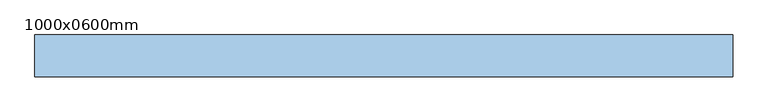
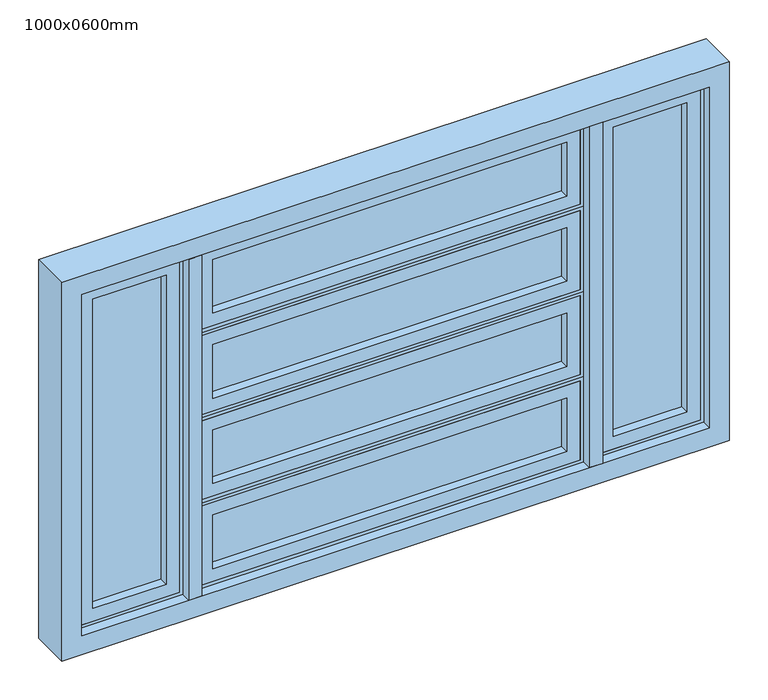
"""IFC4 building model written with IfcOpenShell, lengths in millimetres: window geometry, Janela Basculante 02 : 1000x0600mm."""

from ifc_helpers import new_model, si_unit, frame, origin, place, context, project, spatial, polyline, outline, extrude, faceted_brep, source, transform, mapped, element, save


def window_1000x0600mm_c1d4fbe1(model_context):
    return source(origin(), model_context, "Body", "SolidModel", [
        extrude(outline(polyline([(452.0, -29.6), (452.0, -36.6), (328.0, -36.6), (328.0, -29.6), (452.0, -29.6)])), frame((0.0, 0.0, 598.0), z_axis=(0.0, 0.0, 1.0), x_axis=(1.0, 0.0, 0.0)), (0.0, 0.0, 1.0), 504.0),
        faceted_brep([(335.0, -50.6, 1095.0), (335.0, -50.6, 605.0), (335.0, -36.6, 605.0), (335.0, -36.6, 1095.0), (328.0, -36.6, 1102.0), (328.0, -36.6, 598.0), (328.0, -29.6, 598.0), (328.0, -29.6, 1102.0), (335.0, -29.6, 1095.0), (335.0, -29.6, 605.0), (335.0, -15.6, 605.0), (335.0, -15.6, 1095.0), (315.0, -15.6, 1115.0), (315.0, -15.6, 585.0), (315.0, -50.6, 585.0), (315.0, -50.6, 1115.0), (445.0, -50.6, 605.0), (445.0, -36.6, 605.0), (452.0, -36.6, 598.0), (452.0, -29.6, 598.0), (445.0, -29.6, 605.0), (445.0, -15.6, 605.0), (465.0, -15.6, 585.0), (465.0, -50.6, 585.0), (445.0, -50.6, 1095.0), (445.0, -36.6, 1095.0), (452.0, -36.6, 1102.0), (452.0, -29.6, 1102.0), (445.0, -29.6, 1095.0), (445.0, -15.6, 1095.0), (465.0, -15.6, 1115.0), (465.0, -50.6, 1115.0)], [[[0, 1, 2, 3]], [[4, 5, 6, 7]], [[8, 9, 10, 11]], [[12, 13, 14, 15]], [[1, 16, 17, 2]], [[5, 18, 19, 6]], [[9, 20, 21, 10]], [[13, 22, 23, 14]], [[16, 24, 25, 17]], [[18, 26, 27, 19]], [[20, 28, 29, 21]], [[22, 30, 31, 23]], [[15, 14, 23, 31], [1, 0, 24, 16]], [[24, 0, 3, 25]], [[5, 4, 26, 18], [3, 2, 17, 25]], [[26, 4, 7, 27]], [[7, 6, 19, 27], [9, 8, 28, 20]], [[28, 8, 11, 29]], [[13, 12, 30, 22], [11, 10, 21, 29]], [[30, 12, 15, 31]]]),
        faceted_brep([(315.0, -50.6, 1115.0), (315.0, -50.6, 585.0), (315.0, -15.6, 585.0), (315.0, -15.6, 1115.0), (320.0, -15.6, 1110.0), (320.0, -15.6, 590.0), (320.0, -10.6, 590.0), (320.0, -10.6, 1110.0), (310.0, -10.6, 1120.0), (310.0, -10.6, 580.0), (310.0, -50.6, 580.0), (310.0, -50.6, 1120.0), (465.0, -50.6, 585.0), (465.0, -15.6, 585.0), (460.0, -15.6, 590.0), (460.0, -10.6, 590.0), (470.0, -10.6, 580.0), (470.0, -50.6, 580.0), (465.0, -50.6, 1115.0), (465.0, -15.6, 1115.0), (460.0, -15.6, 1110.0), (460.0, -10.6, 1110.0), (470.0, -10.6, 1120.0), (470.0, -50.6, 1120.0)], [[[0, 1, 2, 3]], [[4, 5, 6, 7]], [[8, 9, 10, 11]], [[1, 12, 13, 2]], [[5, 14, 15, 6]], [[9, 16, 17, 10]], [[12, 18, 19, 13]], [[14, 20, 21, 15]], [[16, 22, 23, 17]], [[11, 10, 17, 23], [1, 0, 18, 12]], [[18, 0, 3, 19]], [[3, 2, 13, 19], [5, 4, 20, 14]], [[20, 4, 7, 21]], [[9, 8, 22, 16], [7, 6, 15, 21]], [[22, 8, 11, 23]]]),
        extrude(outline(polyline([(-452.0, -29.6), (-328.0, -29.6), (-328.0, -36.6), (-452.0, -36.6), (-452.0, -29.6)])), frame((0.0, 0.0, 598.0), z_axis=(0.0, 0.0, 1.0), x_axis=(1.0, 0.0, 0.0)), (0.0, 0.0, 1.0), 504.0),
        faceted_brep([(-335.0, -50.6, 1095.0), (-335.0, -36.6, 1095.0), (-335.0, -36.6, 605.0), (-335.0, -50.6, 605.0), (-328.0, -36.6, 1102.0), (-328.0, -29.6, 1102.0), (-328.0, -29.6, 598.0), (-328.0, -36.6, 598.0), (-335.0, -29.6, 1095.0), (-335.0, -15.6, 1095.0), (-335.0, -15.6, 605.0), (-335.0, -29.6, 605.0), (-315.0, -15.6, 1115.0), (-315.0, -50.6, 1115.0), (-315.0, -50.6, 585.0), (-315.0, -15.6, 585.0), (-445.0, -36.6, 605.0), (-445.0, -50.6, 605.0), (-452.0, -29.6, 598.0), (-452.0, -36.6, 598.0), (-445.0, -15.6, 605.0), (-445.0, -29.6, 605.0), (-465.0, -50.6, 585.0), (-465.0, -15.6, 585.0), (-445.0, -36.6, 1095.0), (-445.0, -50.6, 1095.0), (-452.0, -29.6, 1102.0), (-452.0, -36.6, 1102.0), (-445.0, -15.6, 1095.0), (-445.0, -29.6, 1095.0), (-465.0, -50.6, 1115.0), (-465.0, -15.6, 1115.0)], [[[0, 1, 2, 3]], [[4, 5, 6, 7]], [[8, 9, 10, 11]], [[12, 13, 14, 15]], [[3, 2, 16, 17]], [[7, 6, 18, 19]], [[11, 10, 20, 21]], [[15, 14, 22, 23]], [[17, 16, 24, 25]], [[19, 18, 26, 27]], [[21, 20, 28, 29]], [[23, 22, 30, 31]], [[13, 30, 22, 14], [3, 17, 25, 0]], [[25, 24, 1, 0]], [[7, 19, 27, 4], [1, 24, 16, 2]], [[27, 26, 5, 4]], [[5, 26, 18, 6], [11, 21, 29, 8]], [[29, 28, 9, 8]], [[15, 23, 31, 12], [9, 28, 20, 10]], [[31, 30, 13, 12]]]),
        faceted_brep([(-315.0, -50.6, 1115.0), (-315.0, -15.6, 1115.0), (-315.0, -15.6, 585.0), (-315.0, -50.6, 585.0), (-320.0, -15.6, 1110.0), (-320.0, -10.6, 1110.0), (-320.0, -10.6, 590.0), (-320.0, -15.6, 590.0), (-310.0, -10.6, 1120.0), (-310.0, -50.6, 1120.0), (-310.0, -50.6, 580.0), (-310.0, -10.6, 580.0), (-465.0, -15.6, 585.0), (-465.0, -50.6, 585.0), (-460.0, -10.6, 590.0), (-460.0, -15.6, 590.0), (-470.0, -50.6, 580.0), (-470.0, -10.6, 580.0), (-465.0, -15.6, 1115.0), (-465.0, -50.6, 1115.0), (-460.0, -10.6, 1110.0), (-460.0, -15.6, 1110.0), (-470.0, -50.6, 1120.0), (-470.0, -10.6, 1120.0)], [[[0, 1, 2, 3]], [[4, 5, 6, 7]], [[8, 9, 10, 11]], [[3, 2, 12, 13]], [[7, 6, 14, 15]], [[11, 10, 16, 17]], [[13, 12, 18, 19]], [[15, 14, 20, 21]], [[17, 16, 22, 23]], [[9, 22, 16, 10], [3, 13, 19, 0]], [[19, 18, 1, 0]], [[1, 18, 12, 2], [7, 15, 21, 4]], [[21, 20, 5, 4]], [[11, 17, 23, 8], [5, 20, 14, 6]], [[23, 22, 9, 8]]]),
        extrude(outline(polyline([(-272.0, -29.6), (272.0, -29.6), (272.0, -36.6), (-272.0, -36.6), (-272.0, -29.6)])), frame((0.0, 0.0, 1003.0), z_axis=(0.0, 0.0, 1.0), x_axis=(1.0, 0.0, 0.0)), (0.0, 0.0, 1.0), 99.0),
        faceted_brep([(265.0, -50.6, 1095.0), (265.0, -36.6, 1095.0), (265.0, -36.6, 1010.0), (265.0, -50.6, 1010.0), (272.0, -36.6, 1102.0), (272.0, -29.6, 1102.0), (272.0, -29.6, 1003.0), (272.0, -36.6, 1003.0), (265.0, -29.6, 1095.0), (265.0, -15.6, 1095.0), (265.0, -15.6, 1010.0), (265.0, -29.6, 1010.0), (285.0, -15.6, 1115.0), (285.0, -50.6, 1115.0), (285.0, -50.6, 990.0), (285.0, -15.6, 990.0), (-265.0, -36.6, 1010.0), (-265.0, -50.6, 1010.0), (-272.0, -29.6, 1003.0), (-272.0, -36.6, 1003.0), (-265.0, -15.6, 1010.0), (-265.0, -29.6, 1010.0), (-285.0, -50.6, 990.0), (-285.0, -15.6, 990.0), (-265.0, -36.6, 1095.0), (-265.0, -50.6, 1095.0), (-272.0, -29.6, 1102.0), (-272.0, -36.6, 1102.0), (-265.0, -15.6, 1095.0), (-265.0, -29.6, 1095.0), (-285.0, -50.6, 1115.0), (-285.0, -15.6, 1115.0)], [[[0, 1, 2, 3]], [[4, 5, 6, 7]], [[8, 9, 10, 11]], [[12, 13, 14, 15]], [[3, 2, 16, 17]], [[7, 6, 18, 19]], [[11, 10, 20, 21]], [[15, 14, 22, 23]], [[17, 16, 24, 25]], [[19, 18, 26, 27]], [[21, 20, 28, 29]], [[23, 22, 30, 31]], [[13, 30, 22, 14], [3, 17, 25, 0]], [[25, 24, 1, 0]], [[7, 19, 27, 4], [1, 24, 16, 2]], [[27, 26, 5, 4]], [[5, 26, 18, 6], [11, 21, 29, 8]], [[29, 28, 9, 8]], [[15, 23, 31, 12], [9, 28, 20, 10]], [[31, 30, 13, 12]]]),
        faceted_brep([(285.0, -50.6, 1115.0), (285.0, -15.6, 1115.0), (285.0, -15.6, 990.0), (285.0, -50.6, 990.0), (280.0, -15.6, 1110.0), (280.0, -10.6, 1110.0), (280.0, -10.6, 995.0), (280.0, -15.6, 995.0), (290.0, -10.6, 1120.0), (290.0, -50.6, 1120.0), (290.0, -50.6, 985.0), (290.0, -10.6, 985.0), (-285.0, -15.6, 990.0), (-285.0, -50.6, 990.0), (-280.0, -10.6, 995.0), (-280.0, -15.6, 995.0), (-290.0, -50.6, 985.0), (-290.0, -10.6, 985.0), (-285.0, -15.6, 1115.0), (-285.0, -50.6, 1115.0), (-280.0, -10.6, 1110.0), (-280.0, -15.6, 1110.0), (-290.0, -50.6, 1120.0), (-290.0, -10.6, 1120.0)], [[[0, 1, 2, 3]], [[4, 5, 6, 7]], [[8, 9, 10, 11]], [[3, 2, 12, 13]], [[7, 6, 14, 15]], [[11, 10, 16, 17]], [[13, 12, 18, 19]], [[15, 14, 20, 21]], [[17, 16, 22, 23]], [[9, 22, 16, 10], [3, 13, 19, 0]], [[19, 18, 1, 0]], [[1, 18, 12, 2], [7, 15, 21, 4]], [[21, 20, 5, 4]], [[11, 17, 23, 8], [5, 20, 14, 6]], [[23, 22, 9, 8]]]),
        extrude(outline(polyline([(-272.0, -29.6), (272.0, -29.6), (272.0, -36.6), (-272.0, -36.6), (-272.0, -29.6)])), frame((0.0, 0.0, 868.0), z_axis=(0.0, 0.0, 1.0), x_axis=(1.0, 0.0, 0.0)), (0.0, 0.0, 1.0), 99.0),
        faceted_brep([(265.0, -50.6, 960.0), (265.0, -36.6, 960.0), (265.0, -36.6, 875.0), (265.0, -50.6, 875.0), (272.0, -36.6, 967.0), (272.0, -29.6, 967.0), (272.0, -29.6, 868.0), (272.0, -36.6, 868.0), (265.0, -29.6, 960.0), (265.0, -15.6, 960.0), (265.0, -15.6, 875.0), (265.0, -29.6, 875.0), (285.0, -15.6, 980.0), (285.0, -50.6, 980.0), (285.0, -50.6, 855.0), (285.0, -15.6, 855.0), (-265.0, -36.6, 875.0), (-265.0, -50.6, 875.0), (-272.0, -29.6, 868.0), (-272.0, -36.6, 868.0), (-265.0, -15.6, 875.0), (-265.0, -29.6, 875.0), (-285.0, -50.6, 855.0), (-285.0, -15.6, 855.0), (-265.0, -36.6, 960.0), (-265.0, -50.6, 960.0), (-272.0, -29.6, 967.0), (-272.0, -36.6, 967.0), (-265.0, -15.6, 960.0), (-265.0, -29.6, 960.0), (-285.0, -50.6, 980.0), (-285.0, -15.6, 980.0)], [[[0, 1, 2, 3]], [[4, 5, 6, 7]], [[8, 9, 10, 11]], [[12, 13, 14, 15]], [[3, 2, 16, 17]], [[7, 6, 18, 19]], [[11, 10, 20, 21]], [[15, 14, 22, 23]], [[17, 16, 24, 25]], [[19, 18, 26, 27]], [[21, 20, 28, 29]], [[23, 22, 30, 31]], [[13, 30, 22, 14], [3, 17, 25, 0]], [[25, 24, 1, 0]], [[7, 19, 27, 4], [1, 24, 16, 2]], [[27, 26, 5, 4]], [[5, 26, 18, 6], [11, 21, 29, 8]], [[29, 28, 9, 8]], [[15, 23, 31, 12], [9, 28, 20, 10]], [[31, 30, 13, 12]]]),
        faceted_brep([(285.0, -50.6, 980.0), (285.0, -15.6, 980.0), (285.0, -15.6, 855.0), (285.0, -50.6, 855.0), (280.0, -15.6, 975.0), (280.0, -10.6, 975.0), (280.0, -10.6, 860.0), (280.0, -15.6, 860.0), (290.0, -10.6, 985.0), (290.0, -50.6, 985.0), (290.0, -50.6, 850.0), (290.0, -10.6, 850.0), (-285.0, -15.6, 855.0), (-285.0, -50.6, 855.0), (-280.0, -10.6, 860.0), (-280.0, -15.6, 860.0), (-290.0, -50.6, 850.0), (-290.0, -10.6, 850.0), (-285.0, -15.6, 980.0), (-285.0, -50.6, 980.0), (-280.0, -10.6, 975.0), (-280.0, -15.6, 975.0), (-290.0, -50.6, 985.0), (-290.0, -10.6, 985.0)], [[[0, 1, 2, 3]], [[4, 5, 6, 7]], [[8, 9, 10, 11]], [[3, 2, 12, 13]], [[7, 6, 14, 15]], [[11, 10, 16, 17]], [[13, 12, 18, 19]], [[15, 14, 20, 21]], [[17, 16, 22, 23]], [[9, 22, 16, 10], [3, 13, 19, 0]], [[19, 18, 1, 0]], [[1, 18, 12, 2], [7, 15, 21, 4]], [[21, 20, 5, 4]], [[11, 17, 23, 8], [5, 20, 14, 6]], [[23, 22, 9, 8]]]),
        extrude(outline(polyline([(-272.0, -29.6), (272.0, -29.6), (272.0, -36.6), (-272.0, -36.6), (-272.0, -29.6)])), frame((0.0, 0.0, 733.0), z_axis=(0.0, 0.0, 1.0), x_axis=(1.0, 0.0, 0.0)), (0.0, 0.0, 1.0), 99.0),
        faceted_brep([(265.0, -50.6, 825.0), (265.0, -36.6, 825.0), (265.0, -36.6, 740.0), (265.0, -50.6, 740.0), (272.0, -36.6, 832.0), (272.0, -29.6, 832.0), (272.0, -29.6, 733.0), (272.0, -36.6, 733.0), (265.0, -29.6, 825.0), (265.0, -15.6, 825.0), (265.0, -15.6, 740.0), (265.0, -29.6, 740.0), (285.0, -15.6, 845.0), (285.0, -50.6, 845.0), (285.0, -50.6, 720.0), (285.0, -15.6, 720.0), (-265.0, -36.6, 740.0), (-265.0, -50.6, 740.0), (-272.0, -29.6, 733.0), (-272.0, -36.6, 733.0), (-265.0, -15.6, 740.0), (-265.0, -29.6, 740.0), (-285.0, -50.6, 720.0), (-285.0, -15.6, 720.0), (-265.0, -36.6, 825.0), (-265.0, -50.6, 825.0), (-272.0, -29.6, 832.0), (-272.0, -36.6, 832.0), (-265.0, -15.6, 825.0), (-265.0, -29.6, 825.0), (-285.0, -50.6, 845.0), (-285.0, -15.6, 845.0)], [[[0, 1, 2, 3]], [[4, 5, 6, 7]], [[8, 9, 10, 11]], [[12, 13, 14, 15]], [[3, 2, 16, 17]], [[7, 6, 18, 19]], [[11, 10, 20, 21]], [[15, 14, 22, 23]], [[17, 16, 24, 25]], [[19, 18, 26, 27]], [[21, 20, 28, 29]], [[23, 22, 30, 31]], [[13, 30, 22, 14], [3, 17, 25, 0]], [[25, 24, 1, 0]], [[7, 19, 27, 4], [1, 24, 16, 2]], [[27, 26, 5, 4]], [[5, 26, 18, 6], [11, 21, 29, 8]], [[29, 28, 9, 8]], [[15, 23, 31, 12], [9, 28, 20, 10]], [[31, 30, 13, 12]]]),
        faceted_brep([(285.0, -50.6, 845.0), (285.0, -15.6, 845.0), (285.0, -15.6, 720.0), (285.0, -50.6, 720.0), (280.0, -15.6, 840.0), (280.0, -10.6, 840.0), (280.0, -10.6, 725.0), (280.0, -15.6, 725.0), (290.0, -10.6, 850.0), (290.0, -50.6, 850.0), (290.0, -50.6, 715.0), (290.0, -10.6, 715.0), (-285.0, -15.6, 720.0), (-285.0, -50.6, 720.0), (-280.0, -10.6, 725.0), (-280.0, -15.6, 725.0), (-290.0, -50.6, 715.0), (-290.0, -10.6, 715.0), (-285.0, -15.6, 845.0), (-285.0, -50.6, 845.0), (-280.0, -10.6, 840.0), (-280.0, -15.6, 840.0), (-290.0, -50.6, 850.0), (-290.0, -10.6, 850.0)], [[[0, 1, 2, 3]], [[4, 5, 6, 7]], [[8, 9, 10, 11]], [[3, 2, 12, 13]], [[7, 6, 14, 15]], [[11, 10, 16, 17]], [[13, 12, 18, 19]], [[15, 14, 20, 21]], [[17, 16, 22, 23]], [[9, 22, 16, 10], [3, 13, 19, 0]], [[19, 18, 1, 0]], [[1, 18, 12, 2], [7, 15, 21, 4]], [[21, 20, 5, 4]], [[11, 17, 23, 8], [5, 20, 14, 6]], [[23, 22, 9, 8]]]),
        extrude(outline(polyline([(-272.0, -29.6), (272.0, -29.6), (272.0, -36.6), (-272.0, -36.6), (-272.0, -29.6)])), frame((0.0, 0.0, 598.0), z_axis=(0.0, 0.0, 1.0), x_axis=(1.0, 0.0, 0.0)), (0.0, 0.0, 1.0), 99.0),
        faceted_brep([(265.0, -50.6, 690.0), (265.0, -36.6, 690.0), (265.0, -36.6, 605.0), (265.0, -50.6, 605.0), (272.0, -36.6, 697.0), (272.0, -29.6, 697.0), (272.0, -29.6, 598.0), (272.0, -36.6, 598.0), (265.0, -29.6, 690.0), (265.0, -15.6, 690.0), (265.0, -15.6, 605.0), (265.0, -29.6, 605.0), (285.0, -15.6, 710.0), (285.0, -50.6, 710.0), (285.0, -50.6, 585.0), (285.0, -15.6, 585.0), (-265.0, -36.6, 605.0), (-265.0, -50.6, 605.0), (-272.0, -29.6, 598.0), (-272.0, -36.6, 598.0), (-265.0, -15.6, 605.0), (-265.0, -29.6, 605.0), (-285.0, -50.6, 585.0), (-285.0, -15.6, 585.0), (-265.0, -36.6, 690.0), (-265.0, -50.6, 690.0), (-272.0, -29.6, 697.0), (-272.0, -36.6, 697.0), (-265.0, -15.6, 690.0), (-265.0, -29.6, 690.0), (-285.0, -50.6, 710.0), (-285.0, -15.6, 710.0)], [[[0, 1, 2, 3]], [[4, 5, 6, 7]], [[8, 9, 10, 11]], [[12, 13, 14, 15]], [[3, 2, 16, 17]], [[7, 6, 18, 19]], [[11, 10, 20, 21]], [[15, 14, 22, 23]], [[17, 16, 24, 25]], [[19, 18, 26, 27]], [[21, 20, 28, 29]], [[23, 22, 30, 31]], [[13, 30, 22, 14], [3, 17, 25, 0]], [[25, 24, 1, 0]], [[7, 19, 27, 4], [1, 24, 16, 2]], [[27, 26, 5, 4]], [[5, 26, 18, 6], [11, 21, 29, 8]], [[29, 28, 9, 8]], [[15, 23, 31, 12], [9, 28, 20, 10]], [[31, 30, 13, 12]]]),
        faceted_brep([(285.0, -50.6, 710.0), (285.0, -15.6, 710.0), (285.0, -15.6, 585.0), (285.0, -50.6, 585.0), (280.0, -15.6, 705.0), (280.0, -10.6, 705.0), (280.0, -10.6, 590.0), (280.0, -15.6, 590.0), (290.0, -10.6, 715.0), (290.0, -50.6, 715.0), (290.0, -50.6, 580.0), (290.0, -10.6, 580.0), (-285.0, -15.6, 585.0), (-285.0, -50.6, 585.0), (-280.0, -10.6, 590.0), (-280.0, -15.6, 590.0), (-290.0, -50.6, 580.0), (-290.0, -10.6, 580.0), (-285.0, -15.6, 710.0), (-285.0, -50.6, 710.0), (-280.0, -10.6, 705.0), (-280.0, -15.6, 705.0), (-290.0, -50.6, 715.0), (-290.0, -10.6, 715.0)], [[[0, 1, 2, 3]], [[4, 5, 6, 7]], [[8, 9, 10, 11]], [[3, 2, 12, 13]], [[7, 6, 14, 15]], [[11, 10, 16, 17]], [[13, 12, 18, 19]], [[15, 14, 20, 21]], [[17, 16, 22, 23]], [[9, 22, 16, 10], [3, 13, 19, 0]], [[19, 18, 1, 0]], [[1, 18, 12, 2], [7, 15, 21, 4]], [[21, 20, 5, 4]], [[11, 17, 23, 8], [5, 20, 14, 6]], [[23, 22, 9, 8]]]),
        extrude(outline(polyline([(290.0, -10.6), (310.0, -10.6), (310.0, -65.6), (290.0, -65.6), (290.0, -10.6)])), frame((0.0, 0.0, 580.0), z_axis=(0.0, 0.0, 1.0), x_axis=(1.0, 0.0, 0.0)), (0.0, 0.0, 1.0), 540.0),
        extrude(outline(polyline([(-310.0, -10.6), (-290.0, -10.6), (-290.0, -65.6), (-310.0, -65.6), (-310.0, -10.6)])), frame((0.0, 0.0, 580.0), z_axis=(0.0, 0.0, 1.0), x_axis=(1.0, 0.0, 0.0)), (0.0, 0.0, 1.0), 540.0),
        faceted_brep([(500.0, -5.6, 1150.0), (500.0, -65.6, 1150.0), (500.0, -65.6, 550.0), (500.0, -5.6, 550.0), (-500.0, -65.6, 1150.0), (-500.0, -65.6, 550.0), (470.0, -65.6, 580.0), (-470.0, -65.6, 580.0), (-470.0, -65.6, 1120.0), (470.0, -65.6, 1120.0), (-500.0, -5.6, 550.0), (-500.0, -5.6, 1150.0), (460.0, -5.6, 1110.0), (-460.0, -5.6, 1110.0), (-460.0, -5.6, 590.0), (460.0, -5.6, 590.0), (470.0, -10.6, 1120.0), (470.0, -10.6, 580.0), (-470.0, -10.6, 1120.0), (-470.0, -10.6, 580.0), (460.0, -10.6, 590.0), (-460.0, -10.6, 590.0), (-460.0, -10.6, 1110.0), (460.0, -10.6, 1110.0)], [[[0, 1, 2, 3]], [[1, 4, 5, 2], [6, 7, 8, 9]], [[3, 2, 5, 10]], [[3, 10, 11, 0], [12, 13, 14, 15]], [[9, 16, 17, 6]], [[16, 18, 19, 17], [20, 21, 22, 23]], [[6, 17, 19, 7]], [[10, 5, 4, 11]], [[7, 19, 18, 8]], [[23, 12, 15, 20]], [[20, 15, 14, 21]], [[21, 14, 13, 22]], [[11, 4, 1, 0]], [[8, 18, 16, 9]], [[22, 13, 12, 23]]]),
    ])


if __name__ == "__main__":
    model = new_model("IFC4")
    model_context = context("Model", 3, world=origin())
    ifc_project = project(units=[si_unit("LENGTHUNIT", "METRE", prefix="MILLI")], contexts=[model_context])
    site = spatial("IfcSite", under=ifc_project)
    building = spatial("IfcBuilding", under=site)
    placement = place(None, origin())
    window_1000x0600mm_shape = window_1000x0600mm_c1d4fbe1(model_context)
    element("IfcWindow", 1, ObjectType="Janela Basculante 02 : 1000x0600mm", at=placement, inside=building, context=model_context, shape_type="MappedRepresentation", body=[
        mapped(window_1000x0600mm_shape, transform((0.0, 0.0, 0.0), x_axis=(1.0, 0.0, 0.0), y_axis=(0.0, 1.0, 0.0), z_axis=(0.0, 0.0, 1.0))),
    ])
    save(model, "model.ifc")

# Revit data of these elements
# Type "Janela Basculante 02 : 1000x0600mm"
#   Type Mark = ""
#   SINAPI = ""
#   ref. v bascula = 13.50 cm
#   ref. h bascula = 58.00 cm
#   Ref. h basc lateral = 16.00 cm
#   Módulo Básico M = 10.00 cm
#   Largura de Coordenação Modular CM = 100.00 cm
#   Largura bascula lateral = 20.00 cm
#   Largura Batente = 6.00 cm
#   Altura de Coordenação Modular CM = 60.00 cm
#   Height = 60.00 cm
#   Altura Peitoril = 55.00 cm
#   Width = 100.00 cm
#   Altura Bascula Lateral = 54.00 cm
#   n° de basculas = 4
#   Número de Módulos Básicos nM Largura = 10
#   Número de Módulos Básicos nM Altura = 6
#   Material Quadro = Metal - Alumínio
#   Material Painel = Vidro
#   Wall Closure = (empty or 0)
#   Assembly Code = ""
# Element 1 (IfcWindow, "Janela Basculante 02 : 1000x0600mm")
#   Materials on its faces: "Metal - Alumínio", "Vidro"
# Materials
#   "Metal - Alumínio": class "Metal", colour RGB 244 244 244, transparency 0
#   "Vidro": class "Vidro", colour RGB 230 230 230, transparency 0.75, Cost = 0
